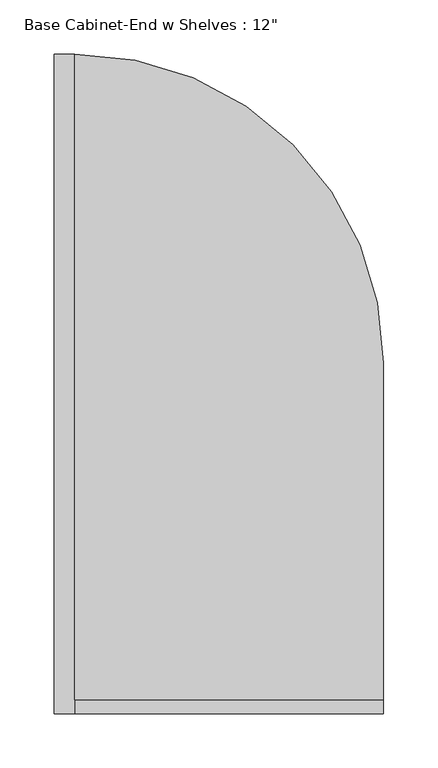
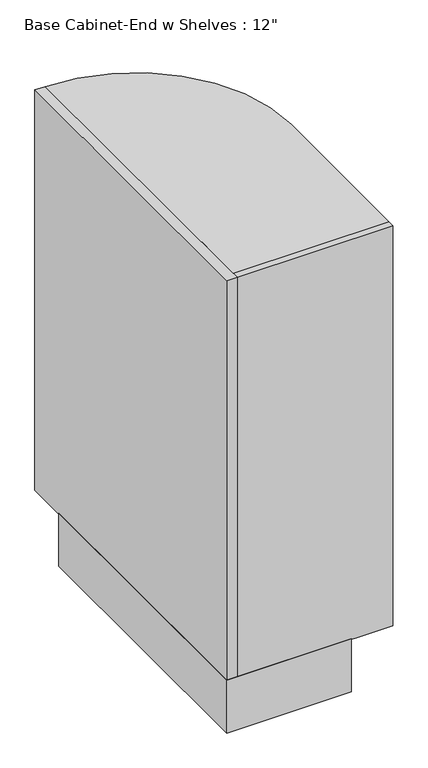
"""IFC4 building model written with IfcOpenShell, lengths in millimetres: furniture geometry."""

from ifc_helpers import new_model, si_unit, point, frame, frame_2d, origin, origin_with_axes, place, context, project, spatial, polyline, circle_curve, trimmed, segment, composite_curve, outline, extrude, source, transform, mapped, element, save


def furniture_38852b6a(model_context):
    return source(origin(), model_context, "Body", "SweptSolid", [
        extrude(outline(composite_curve([segment(polyline([(228.6, 0.0), (0.0, 0.0), (0.0, 533.4), (19.0500002, 533.4)]), True, "CONTINUOUS"), segment(trimmed(circle_curve(frame_2d((19.0500002, 323.8500002)), 209.5499998), [point((19.0500002, 533.4))], [point((228.6, 323.8500002))], False, "CARTESIAN"), True, "CONTINUOUS"), segment(polyline([(228.6, 323.8500002), (228.6, 0.0)]), True, "CONTINUOUS")], self_intersect=False)), origin_with_axes(), (0.0, 0.0, 1.0), 102.790625),
        extrude(outline(composite_curve([segment(polyline([(304.8, 12.7), (19.05, 12.7), (19.05, 609.5999998)]), True, "CONTINUOUS"), segment(trimmed(circle_curve(frame_2d((19.05, 323.8499999)), 285.75), [point((19.05, 609.5999998))], [point((304.8, 323.8499999))], False, "CARTESIAN"), True, "CONTINUOUS"), segment(polyline([(304.8, 323.8499999), (304.8, 12.7)]), True, "CONTINUOUS")], self_intersect=False)), frame((0.0, 0.0, 102.790625), z_axis=(0.0, 0.0, 1.0), x_axis=(1.0, 0.0, 0.0)), (0.0, 0.0, 1.0), 19.05),
        extrude(outline(composite_curve([segment(polyline([(19.05, 12.7), (19.05, 609.6)]), True, "CONTINUOUS"), segment(trimmed(circle_curve(frame_2d((19.05, 323.85)), 285.75), [point((19.05, 609.6))], [point((304.8, 323.85))], False, "CARTESIAN"), True, "CONTINUOUS"), segment(polyline([(304.8, 323.85), (304.8, 12.7), (19.05, 12.7)]), True, "CONTINUOUS")], self_intersect=False)), frame((0.0, 0.0, 858.440625), z_axis=(0.0, 0.0, 1.0), x_axis=(1.0, 0.0, 0.0)), (0.0, 0.0, 1.0), 19.05),
        extrude(outline(polyline([(0.0, 0.0), (0.0, 609.6), (19.05, 609.6), (19.05, 0.0), (0.0, 0.0)])), frame((0.0, 0.0, 101.6), z_axis=(0.0, 0.0, 1.0), x_axis=(1.0, 0.0, 0.0)), (0.0, 0.0, 1.0), 775.890625),
        extrude(outline(polyline([(304.8, 0.0), (19.05, 0.0), (19.05, 12.7), (304.8, 12.7), (304.8, 0.0)])), frame((0.0, 0.0, 101.6), z_axis=(0.0, 0.0, 1.0), x_axis=(1.0, 0.0, 0.0)), (0.0, 0.0, 1.0), 775.890625),
        extrude(outline(composite_curve([segment(polyline([(304.8, 12.7), (19.05, 12.7), (19.05, 609.6)]), True, "CONTINUOUS"), segment(trimmed(circle_curve(frame_2d((19.05, 323.85)), 285.75), [point((19.05, 609.6))], [point((304.8, 323.85))], False, "CARTESIAN"), True, "CONTINUOUS"), segment(polyline([(304.8, 323.85), (304.8, 12.7)]), True, "CONTINUOUS")], self_intersect=False)), frame((0.0, 0.0, 480.615625), z_axis=(0.0, 0.0, 1.0), x_axis=(1.0, 0.0, 0.0)), (0.0, 0.0, 1.0), 19.05),
    ])


if __name__ == "__main__":
    model = new_model("IFC4")
    model_context = context("Model", 3, world=origin())
    ifc_project = project(units=[si_unit("LENGTHUNIT", "METRE", prefix="MILLI")], contexts=[model_context])
    site = spatial("IfcSite", under=ifc_project)
    building = spatial("IfcBuilding", under=site)
    placement = place(None, origin())
    furniture_shape = furniture_38852b6a(model_context)
    element("IfcFurniture", 1, ObjectType="Base Cabinet-End w Shelves : 12\"", at=placement, inside=building, context=model_context, shape_type="MappedRepresentation", body=[
        mapped(furniture_shape, transform((0.0, 0.0, 0.0), x_axis=(1.0, 0.0, 0.0), y_axis=(0.0, 1.0, 0.0), z_axis=(0.0, 0.0, 1.0))),
    ])
    save(model, "model.ifc")

# Revit data of these elements
# Type "Base Cabinet-End w Shelves : 12\""
#   COBie.Type.CreatedBy = "doug.wood@us.ibm.com"
#   COBie.Type.CreatedOn = "2016-04-14T02:14:45"
#   COBie.Type.Name = "Casework_Base Cabinet-End w Shelves_12\""
#   COBie.Type.Category = "C1030410"
#   COBie.Type.Description = "Base Cabinet-End w Shelves_12\""
#   COBie.Type.Manufacturer = ""
#   COBie.Type.ModelNumber = ""
#   Assembly Code = "C1030410"
#   COBie.Type.ReplacementCost = 0
#   Width = 1' - 0"
#   Toe Kick Depth = 0' - 3"
#   Height = 2' - 10 1/2"
#   Depth = 2' - 0"
#   COBie.Type = no
#   Cabinet Material = Cabinets
# Element 1 (IfcFurniture, "Base Cabinet-End w Shelves : 12\"")
#   Materials on its faces: "Cabinets"
# Materials
#   "Cabinets": class "Miscellaneous", colour RGB 249 249 249, transparency 0
